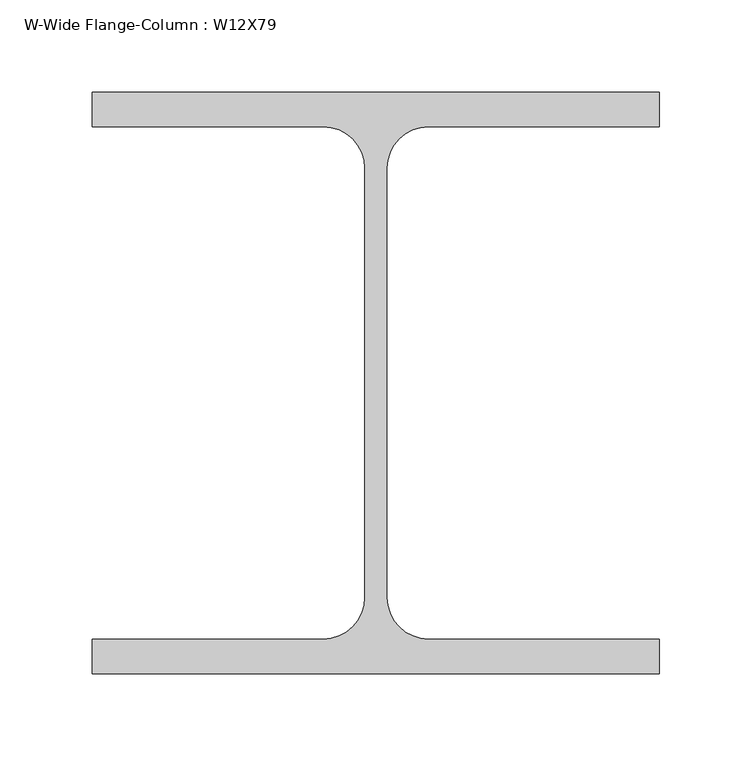
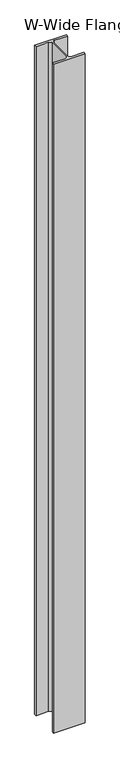
"""IFC4 building model written with IfcOpenShell, lengths in millimetres: column geometry, W-Wide Flange-Column : W12X79."""

import ifcopenshell
import ifcopenshell.guid

model = None  # the IFC model being written
_history = None  # IfcOwnerHistory: only IFC2X3 demands one
_inside = {}  # id of a spatial element -> (the spatial element, [elements in it])
_under = {}  # id of a project, library or spatial element -> (it, [spatial elements below it])
_declared = {}  # id of a project -> (the project, [libraries it declares])
_typed = {}  # id of a type object -> (the type object, [elements of that type])
_made_of = {}  # id of a material, layer set ... -> (it, [elements and type objects made of it])


def new_model(schema):
    """Start an empty IFC model of exactly this schema.

    Asked for "IFC4X3", IfcOpenShell would pick the latest addendum, in which some entities
    have other attributes; the version numbers below select the first issue.
    IFC2X3 requires an IfcOwnerHistory on every rooted entity: one is made here for all.
    """
    global model, _history
    if schema == "IFC4X3":
        model = ifcopenshell.file(schema_version=(4, 3, 0, 0))
    else:
        model = ifcopenshell.file(schema=schema)
    _inside.clear()
    _under.clear()
    _declared.clear()
    _typed.clear()
    _made_of.clear()
    _history = None
    if model.schema == "IFC2X3":
        org = make("IfcOrganization", Name="unknown")
        user = make(
            "IfcPersonAndOrganization",
            ThePerson=make("IfcPerson", FamilyName="unknown"),
            TheOrganization=org,
        )
        app = make(
            "IfcApplication",
            ApplicationDeveloper=org,
            Version="unknown",
            ApplicationFullName="unknown",
            ApplicationIdentifier="unknown",
        )
        _history = make(
            "IfcOwnerHistory",
            OwningUser=user,
            OwningApplication=app,
            ChangeAction="ADDED",
            CreationDate=0,
        )
    return model


def make(cls, **values):
    """One entity of the class cls with the attributes given. An attribute that is None is left unset."""
    return model.create_entity(
        cls, **{name: value for name, value in values.items() if value is not None}
    )


def rooted(cls, **values):
    """An entity with a GlobalId (a new one), such as an element, a storey or a relation."""
    return make(cls, GlobalId=ifcopenshell.guid.new(), OwnerHistory=_history, **values)


def si_unit(unit_type, name, prefix=None):
    """IfcSIUnit, for example si_unit("LENGTHUNIT", "METRE", prefix="MILLI")."""
    return make("IfcSIUnit", UnitType=unit_type, Prefix=prefix, Name=name)


def assignment(units):
    """IfcUnitAssignment: the units of a project."""
    return None if units is None else make("IfcUnitAssignment", Units=units)


def point(xyz):
    """IfcCartesianPoint."""
    return None if xyz is None else make("IfcCartesianPoint", Coordinates=xyz)


def direction(xyz):
    """IfcDirection."""
    return None if xyz is None else make("IfcDirection", DirectionRatios=xyz)


def frame(location, z_axis=None, x_axis=None):
    """IfcAxis2Placement3D, a coordinate frame: its origin and axes. An axis left out is left unset."""
    return make(
        "IfcAxis2Placement3D",
        Location=point(location),
        Axis=direction(z_axis),
        RefDirection=direction(x_axis),
    )


def frame_2d(location, x_axis=None):
    """IfcAxis2Placement2D, a coordinate frame in the plane: its origin and x axis."""
    return make(
        "IfcAxis2Placement2D", Location=point(location), RefDirection=direction(x_axis)
    )


def origin():
    """The frame at (0, 0, 0) with its axes left unset."""
    return frame((0.0, 0.0, 0.0))


def place(relative_to, where):
    """IfcLocalPlacement: puts the frame where relative to a parent placement (None: the world)."""
    return make(
        "IfcLocalPlacement", PlacementRelTo=relative_to, RelativePlacement=where
    )


def context(
    kind, dimensions, precision=None, world=None, true_north=None, identifier=None
):
    """IfcGeometricRepresentationContext, for example the 3D "Model" context."""
    return make(
        "IfcGeometricRepresentationContext",
        ContextIdentifier=identifier,
        ContextType=kind,
        CoordinateSpaceDimension=dimensions,
        Precision=precision,
        WorldCoordinateSystem=world,
        TrueNorth=true_north,
    )


def project(units=None, contexts=None):
    """IfcProject with its units and contexts."""
    return rooted(
        "IfcProject",
        Name="project",
        RepresentationContexts=contexts,
        UnitsInContext=assignment(units),
    )


def spatial(cls, under=None, at=None, **own):
    """A site, building, storey or space (cls), placed at a placement, below another one or the project."""
    s = rooted(cls, ObjectPlacement=at, **own)
    if under is not None:
        _under.setdefault(under.id(), (under, []))[1].append(s)
    return s


def polyline(points):
    """IfcPolyline through the points."""
    return make("IfcPolyline", Points=[point(p) for p in points])


def circle_curve(where, radius):
    """IfcCircle in the frame where."""
    return make("IfcCircle", Position=where, Radius=radius)


def trimmed(basis, trim1, trim2, sense, master):
    """IfcTrimmedCurve: the piece of a basis curve between two trims."""
    return make(
        "IfcTrimmedCurve",
        BasisCurve=basis,
        Trim1=trim1,
        Trim2=trim2,
        SenseAgreement=sense,
        MasterRepresentation=master,
    )


def segment(curve, same_sense, transition):
    """IfcCompositeCurveSegment."""
    return make(
        "IfcCompositeCurveSegment",
        Transition=transition,
        SameSense=same_sense,
        ParentCurve=curve,
    )


def composite_curve(segments, self_intersect=None):
    """IfcCompositeCurve: segments joined end to end."""
    return make("IfcCompositeCurve", Segments=segments, SelfIntersect=self_intersect)


def outline(outer, holes=None, kind="AREA"):
    """IfcArbitraryClosedProfileDef: a profile drawn as a closed curve; with holes, ...WithVoids."""
    if holes is None:
        return make("IfcArbitraryClosedProfileDef", ProfileType=kind, OuterCurve=outer)
    return make(
        "IfcArbitraryProfileDefWithVoids",
        ProfileType=kind,
        OuterCurve=outer,
        InnerCurves=holes,
    )


def extrude(swept, where, along, depth):
    """IfcExtrudedAreaSolid: the profile swept, set in the frame where, extruded along a direction by depth."""
    return make(
        "IfcExtrudedAreaSolid",
        SweptArea=swept,
        Position=where,
        ExtrudedDirection=direction(along),
        Depth=depth,
    )


def shape(context_of_items, identifier, shape_type, items):
    """IfcShapeRepresentation: the items that make up one representation, for example the "Body"."""
    return make(
        "IfcShapeRepresentation",
        ContextOfItems=context_of_items,
        RepresentationIdentifier=identifier,
        RepresentationType=shape_type,
        Items=items,
    )


def source(mapping_origin, context_of_items, identifier, shape_type, items):
    """IfcRepresentationMap: a shape defined once, which mapped items show again and again."""
    return make(
        "IfcRepresentationMap",
        MappingOrigin=mapping_origin,
        MappedRepresentation=shape(context_of_items, identifier, shape_type, items),
    )


def transform(
    local_origin,
    x_axis=None,
    y_axis=None,
    z_axis=None,
    scale=None,
    scale2=None,
    scale3=None,
    uniform=True,
):
    """IfcCartesianTransformationOperator3D, or its non-uniform kind. x_axis, y_axis, z_axis: its Axis1, 2, 3."""
    if uniform:
        return make(
            "IfcCartesianTransformationOperator3D",
            Axis1=direction(x_axis),
            Axis2=direction(y_axis),
            LocalOrigin=point(local_origin),
            Scale=scale,
            Axis3=direction(z_axis),
        )
    return make(
        "IfcCartesianTransformationOperator3DnonUniform",
        Axis1=direction(x_axis),
        Axis2=direction(y_axis),
        LocalOrigin=point(local_origin),
        Scale=scale,
        Axis3=direction(z_axis),
        Scale2=scale2,
        Scale3=scale3,
    )


def mapped(mapping_source, mapping_target):
    """IfcMappedItem: shows the shape of a source again, moved by a transform."""
    return make(
        "IfcMappedItem", MappingSource=mapping_source, MappingTarget=mapping_target
    )


def made_of(thing, what):
    """Note that an element or type object is made of a material, layer set ...; save() writes the relation."""
    if what is not None:
        _made_of.setdefault(what.id(), (what, []))[1].append(thing)
    return thing


def element(
    cls,
    number,
    at=None,
    inside=None,
    cuts=None,
    type_object=None,
    material=None,
    context=None,
    identifier="Body",
    shape_type=None,
    held_by="IfcProductDefinitionShape",
    body=None,
    shapes=None,
    **own,
):
    """One element of the class cls, such as IfcWall. Its Tag is "e" and its number.

    at: its placement. inside: the storey or other place that contains it. cuts: it is an
    opening in that element (IfcRelVoidsElement). A single representation is given by context,
    identifier, shape_type and body (its items); several are given by shapes. held_by: the class
    of the entity that holds the representations. save() writes the other relations.
    """
    e = rooted(cls, Tag="e%d" % number, ObjectPlacement=at, **own)
    if body is not None:
        shapes = [shape(context, identifier, shape_type, body)]
    if shapes is not None:
        e.Representation = make(held_by, Representations=shapes)
    if inside is not None:
        _inside.setdefault(inside.id(), (inside, []))[1].append(e)
    if cuts is not None:
        rooted(
            "IfcRelVoidsElement", RelatingBuildingElement=cuts, RelatedOpeningElement=e
        )
    if type_object is not None:
        _typed.setdefault(type_object.id(), (type_object, []))[1].append(e)
    return made_of(e, material)


def aggregate(whole, parts):
    """IfcRelAggregates: a whole, such as a stair, and the parts it consists of."""
    return rooted("IfcRelAggregates", RelatingObject=whole, RelatedObjects=parts)


def save(model, path):
    """Write the relations noted so far, then the file.

    IfcRelAggregates (storeys below a building ...), IfcRelContainedInSpatialStructure (elements
    in a storey), IfcRelDefinesByType, IfcRelAssociatesMaterial and IfcRelDeclares: one each for
    every whole, place, type object, material and project.
    """
    for whole, parts in _under.values():
        aggregate(whole, parts)
    for where, things in _inside.values():
        rooted(
            "IfcRelContainedInSpatialStructure",
            RelatedElements=things,
            RelatingStructure=where,
        )
    for kind, things in _typed.values():
        rooted("IfcRelDefinesByType", RelatedObjects=things, RelatingType=kind)
    for what, things in _made_of.values():
        rooted("IfcRelAssociatesMaterial", RelatedObjects=things, RelatingMaterial=what)
    for by, libraries in _declared.values():
        rooted("IfcRelDeclares", RelatingContext=by, RelatedDefinitions=libraries)
    model.write(path)


def w_wide_flange_column_w12x79_acbb4a60(model_context):
    return source(origin(), model_context, "Body", "SweptSolid", [
        extrude(outline(composite_curve([segment(polyline([(153.67, 157.48), (153.67, 138.811), (28.575, 138.811)]), True, "CONTINUOUS"), segment(trimmed(circle_curve(frame_2d((28.575, 116.205)), 22.606), [point((28.575, 138.811))], [point((5.969, 116.205))], True, "CARTESIAN"), True, "CONTINUOUS"), segment(polyline([(5.969, 116.205), (5.969, -116.205)]), True, "CONTINUOUS"), segment(trimmed(circle_curve(frame_2d((28.575, -116.205)), 22.606), [point((5.969, -116.205))], [point((28.575, -138.811))], True, "CARTESIAN"), True, "CONTINUOUS"), segment(polyline([(28.575, -138.811), (153.67, -138.811), (153.67, -157.48), (-153.67, -157.48), (-153.67, -138.811), (-28.575, -138.811)]), True, "CONTINUOUS"), segment(trimmed(circle_curve(frame_2d((-28.575, -116.205)), 22.606), [point((-28.575, -138.811))], [point((-5.969, -116.205))], True, "CARTESIAN"), True, "CONTINUOUS"), segment(polyline([(-5.969, -116.205), (-5.969, 116.205)]), True, "CONTINUOUS"), segment(trimmed(circle_curve(frame_2d((-28.575, 116.205)), 22.606), [point((-5.969, 116.205))], [point((-28.575, 138.811))], True, "CARTESIAN"), True, "CONTINUOUS"), segment(polyline([(-28.575, 138.811), (-153.67, 138.811), (-153.67, 157.48), (153.67, 157.48)]), True, "CONTINUOUS")], self_intersect=False)), frame((0.0, 0.0, 8756.65), z_axis=(0.0, 0.0, 1.0), x_axis=(1.0, 0.0, 0.0)), (0.0, 0.0, 1.0), 6842.125),
    ])


if __name__ == "__main__":
    model = new_model("IFC4")
    model_context = context("Model", 3, world=origin())
    ifc_project = project(units=[si_unit("LENGTHUNIT", "METRE", prefix="MILLI")], contexts=[model_context])
    site = spatial("IfcSite", under=ifc_project)
    building = spatial("IfcBuilding", under=site)
    placement = place(None, origin())
    w_wide_flange_column_w12x79_shape = w_wide_flange_column_w12x79_acbb4a60(model_context)
    element("IfcColumn", 1, ObjectType="W-Wide Flange-Column : W12X79", at=placement, inside=building, context=model_context, shape_type="MappedRepresentation", body=[
        mapped(w_wide_flange_column_w12x79_shape, transform((0.0, 0.0, 0.0), x_axis=(1.0, 0.0, 0.0), y_axis=(0.0, 1.0, 0.0), z_axis=(0.0, 0.0, 1.0))),
    ])
    save(model, "model.ifc")

# Revit data of these elements
# Type "W-Wide Flange-Column : W12X79"
#   Assembly Code = "B10"
#   W = 79
#   bf = 1' - 0.1"
#   d = 1' - 0.4"
#   k = 0' - 1 5/8"
#   kr = 0' - 0.89"
#   tf = 0' - 0.735"
#   tw = 0' - 0.47"
#   A = 0.161111 SF
#   Structural Material [instance default] = Steel ASTM A992
# Element 1 (IfcColumn, "W-Wide Flange-Column : W12X79")
#   Materials on its faces: "Steel ASTM A992"
# Materials
#   "Steel ASTM A992": class "Metal", colour RGB 199 199 199, transparency 0, Description = "Structural steel 50ksi", Cost = 0
